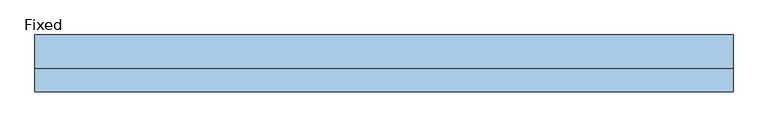
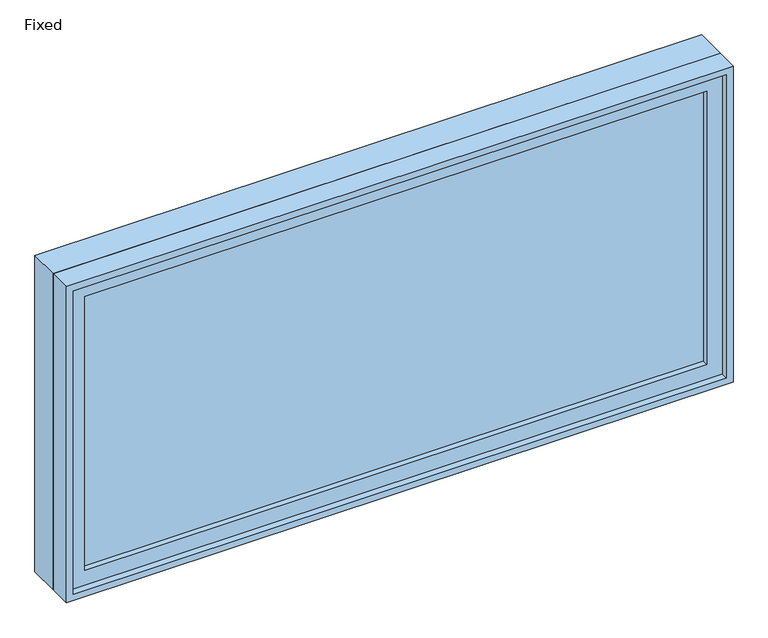
"""IFC4 building model written with IfcOpenShell, lengths in millimetres: window geometry, Fixed."""

from ifc_helpers import new_model, si_unit, frame, origin, place, context, project, spatial, polyline, outline, extrude, source, transform, mapped, element, save


def fixed_4fc4e264(model_context):
    return source(origin(), model_context, "Body", "SweptSolid", [
        extrude(outline(polyline([(835.025, -28.575), (835.025, -41.275), (-911.225, -41.275), (-911.225, -28.575), (835.025, -28.575)])), frame((0.0, 0.0, 1257.3), z_axis=(0.0, 0.0, 1.0), x_axis=(1.0, 0.0, 0.0)), (0.0, 0.0, 1.0), 812.8),
        extrude(outline(polyline([(2114.55, -955.675), (1212.85, -955.675), (1212.85, 879.475), (2114.55, 879.475), (2114.55, -955.675)]), holes=[polyline([(2070.1, -911.225), (2070.1, 835.025), (1257.3, 835.025), (1257.3, -911.225), (2070.1, -911.225)])]), frame((0.0, -57.15, 0.0), z_axis=(0.0, 1.0, 0.0), x_axis=(0.0, 0.0, 1.0)), (0.0, 0.0, 1.0), 44.45),
        extrude(outline(polyline([(2133.6, -974.725), (1193.8, -974.725), (1193.8, 898.525), (2133.6, 898.525), (2133.6, -974.725)]), holes=[polyline([(2101.85, -942.975), (2101.85, 866.775), (1225.55, 866.775), (1225.55, -942.975), (2101.85, -942.975)])]), frame((0.0, -12.7, 0.0), z_axis=(0.0, 1.0, 0.0), x_axis=(0.0, 0.0, 1.0)), (0.0, 0.0, 1.0), 88.9),
        extrude(outline(polyline([(2133.6, 898.525), (2133.6, -974.725), (1193.8, -974.725), (1193.8, 898.525), (2133.6, 898.525)]), holes=[polyline([(2114.55, 879.475), (1212.85, 879.475), (1212.85, -955.675), (2114.55, -955.675), (2114.55, 879.475)])]), frame((0.0, -76.2, 0.0), z_axis=(0.0, 1.0, 0.0), x_axis=(0.0, 0.0, 1.0)), (0.0, 0.0, 1.0), 63.5),
    ])


if __name__ == "__main__":
    model = new_model("IFC4")
    model_context = context("Model", 3, world=origin())
    ifc_project = project(units=[si_unit("LENGTHUNIT", "METRE", prefix="MILLI")], contexts=[model_context])
    site = spatial("IfcSite", under=ifc_project)
    building = spatial("IfcBuilding", under=site)
    placement = place(None, origin())
    fixed_shape = fixed_4fc4e264(model_context)
    element("IfcWindow", 1, ObjectType="Fixed : 6' 1 34\"\" x 3' 1\"", at=placement, inside=building, context=model_context, shape_type="MappedRepresentation", body=[
        mapped(fixed_shape, transform((0.0, 0.0, 0.0), x_axis=(1.0, 0.0, 0.0), y_axis=(0.0, 1.0, 0.0), z_axis=(0.0, 0.0, 1.0))),
    ])
    save(model, "model.ifc")

# Revit data of these elements
# Type "Fixed : 6' 1 34\"\" x 3' 1\""
#   Type Mark = "10"
#   Assembly Code = "B2020100"
#   Height = 3' - 1"
#   Default Sill Height = 3' - 11"
#   Width = 6' - 1 3/4"
#   Window Inset = 0' - 0 3/4"
#   Glass Pane Material = Glass
#   Sash Material = Sash
#   Wall Closure = (empty or 0)
# Element 1 (IfcWindow, "Fixed : 6' 1 34\"\" x 3' 1\"")
#   Materials on its faces: "Sash", "Glass"
# Materials
#   "Glass": class "Glass", colour RGB 218 227 224, transparency 0.85, Description = "Soda Lime Glass", Cost = 0
#   "Sash": class "Wood", colour RGB 136 99 55, transparency 0
